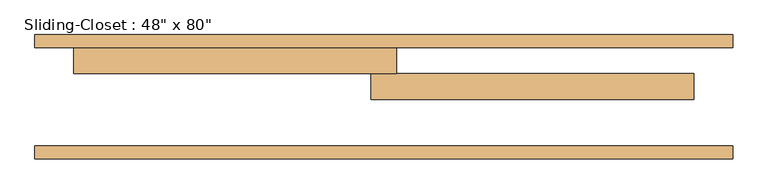
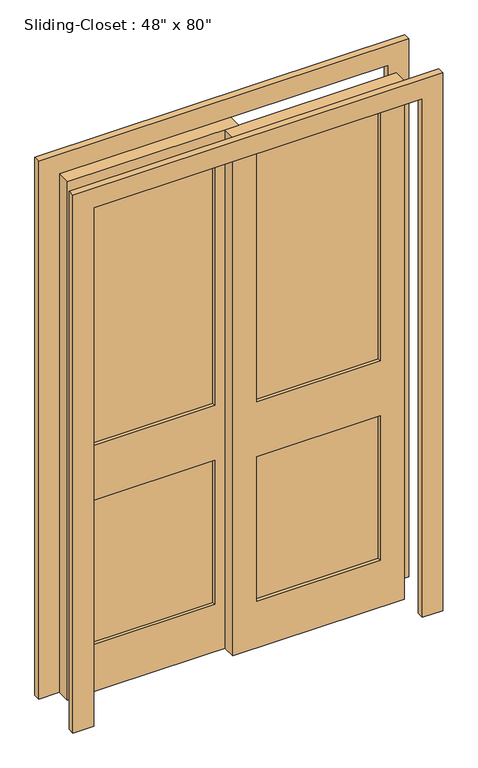
"""IFC4 building model written with IfcOpenShell, lengths in millimetres: door geometry."""

from ifc_helpers import new_model, si_unit, frame, origin, place, context, project, spatial, polyline, outline, extrude, source, transform, mapped, element, save


def door_4b033f1d(model_context):
    return source(origin(), model_context, "Body", "SweptSolid", [
        extrude(outline(polyline([(-63.5, 185.7375), (-520.7, 185.7375), (-520.7, 211.1375), (-63.5, 211.1375), (-63.5, 185.7375)])), frame((0.0, 0.0, 965.2), z_axis=(0.0, 0.0, 1.0), x_axis=(1.0, 0.0, 0.0)), (0.0, 0.0, 1.0), 977.9),
        extrude(outline(polyline([(-63.5, 185.7375), (-520.7, 185.7375), (-520.7, 211.1375), (-63.5, 211.1375), (-63.5, 185.7375)])), frame((0.0, 0.0, 184.15), z_axis=(0.0, 0.0, 1.0), x_axis=(1.0, 0.0, 0.0)), (0.0, 0.0, 1.0), 565.15),
        extrude(outline(polyline([(63.5, 160.3375), (520.7, 160.3375), (520.7, 134.9375), (63.5, 134.9375), (63.5, 160.3375)])), frame((0.0, 0.0, 965.2), z_axis=(0.0, 0.0, 1.0), x_axis=(1.0, 0.0, 0.0)), (0.0, 0.0, 1.0), 977.9),
        extrude(outline(polyline([(63.5, 160.3375), (520.7, 160.3375), (520.7, 134.9375), (63.5, 134.9375), (63.5, 160.3375)])), frame((0.0, 0.0, 184.15), z_axis=(0.0, 0.0, 1.0), x_axis=(1.0, 0.0, 0.0)), (0.0, 0.0, 1.0), 565.15),
        extrude(outline(polyline([(2032.0, 25.4), (2032.0, -609.6), (0.0, -609.6), (0.0, 25.4), (2032.0, 25.4)]), holes=[polyline([(184.15, -520.7), (749.3, -520.7), (749.3, -63.5), (184.15, -63.5), (184.15, -520.7)]), polyline([(965.2, -520.7), (1943.1, -520.7), (1943.1, -63.5), (965.2, -63.5), (965.2, -520.7)])]), frame((0.0, 173.0375, 0.0), z_axis=(0.0, 1.0, 0.0), x_axis=(0.0, 0.0, 1.0)), (0.0, 0.0, 1.0), 50.8),
        extrude(outline(polyline([(0.0, -685.8), (0.0, -609.6), (2032.0, -609.6), (2032.0, 609.6), (0.0, 609.6), (0.0, 685.8), (2108.2, 685.8), (2108.2, -685.8), (0.0, -685.8)])), frame((0.0, 4.7625, 0.0), z_axis=(0.0, 1.0, 0.0), x_axis=(0.0, 0.0, 1.0)), (0.0, 0.0, 1.0), 25.4),
        extrude(outline(polyline([(0.0, 685.8), (2108.2, 685.8), (2108.2, -685.8), (0.0, -685.8), (0.0, -609.6), (2032.0, -609.6), (2032.0, 609.6), (0.0, 609.6), (0.0, 685.8)])), frame((0.0, 223.8375, 0.0), z_axis=(0.0, 1.0, 0.0), x_axis=(0.0, 0.0, 1.0)), (0.0, 0.0, 1.0), 25.4),
        extrude(outline(polyline([(2032.0, -25.4), (0.0, -25.4), (0.0, 609.6), (2032.0, 609.6), (2032.0, -25.4)]), holes=[polyline([(965.2, 520.7), (965.2, 63.5), (1943.1, 63.5), (1943.1, 520.7), (965.2, 520.7)]), polyline([(184.15, 520.7), (184.15, 63.5), (749.3, 63.5), (749.3, 520.7), (184.15, 520.7)])]), frame((0.0, 122.2375, 0.0), z_axis=(0.0, 1.0, 0.0), x_axis=(0.0, 0.0, 1.0)), (0.0, 0.0, 1.0), 50.8),
    ])


if __name__ == "__main__":
    model = new_model("IFC4")
    model_context = context("Model", 3, world=origin())
    ifc_project = project(units=[si_unit("LENGTHUNIT", "METRE", prefix="MILLI")], contexts=[model_context])
    site = spatial("IfcSite", under=ifc_project)
    building = spatial("IfcBuilding", under=site)
    placement = place(None, origin())
    door_shape = door_4b033f1d(model_context)
    element("IfcDoor", 1, ObjectType="Sliding-Closet : 48\" x 80\"", at=placement, inside=building, context=model_context, shape_type="MappedRepresentation", body=[
        mapped(door_shape, transform((0.0, 0.0, 0.0), x_axis=(1.0, 0.0, 0.0), y_axis=(0.0, 1.0, 0.0), z_axis=(0.0, 0.0, 1.0))),
    ])
    save(model, "model.ifc")

# Revit data of these elements
# Type "Sliding-Closet : 48\" x 80\""
#   Type Mark = "54"
#   Assembly Code = "C1020"
#   Thickness = 0' - 2"
#   Height = 6' - 8"
#   Trim Projection Ext = 0' - 1"
#   Trim Projection Int = 0' - 1"
#   Trim Width = 0' - 3"
#   Width = 4' - 0"
#   Define Thermal Properties by = 0
#   Function = 0
#   Door Material = Door - Panel
#   Frame Material = Door - Frame
#   Wall Closure = (empty or 0)
# Element 1 (IfcDoor, "Sliding-Closet : 48\" x 80\"")
#   Materials on its faces: "Door - Panel", "Door - Frame"
# Materials
#   "Door - Panel": class "Wood", colour RGB 227 170 128, transparency 0, Cost = 0
#   "Door - Frame": class "Miscellaneous", colour RGB 153 76 43, transparency 0, Cost = 0
